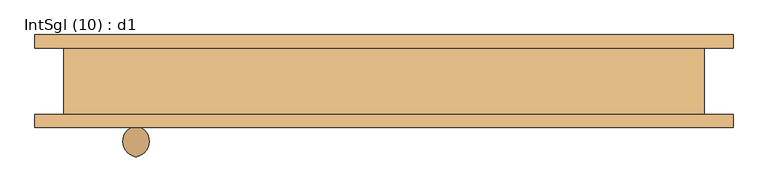
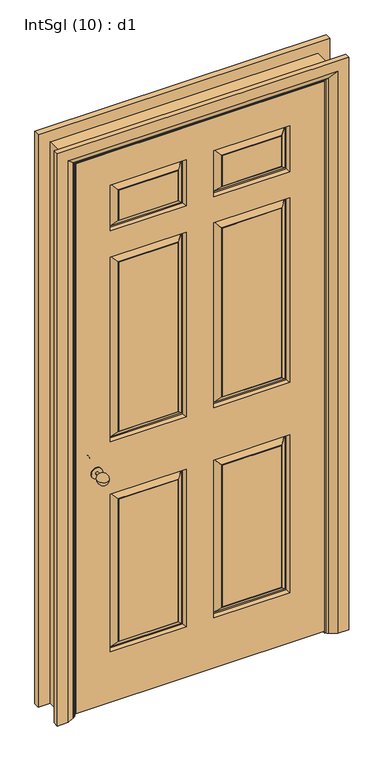
"""IFC4 building model written with IfcOpenShell, lengths in millimetres: door geometry, IntSgl (10) : d1."""

from ifc_helpers import new_model, si_unit, point, frame, origin, place, context, project, spatial, polyline, circle_curve, ellipse_curve, trimmed, outline, extrude, faceted_brep, source, transform, mapped, element, save
from ifc_brep_helpers import plane_surface, cylinder_surface, revolved_surface, advanced_brep


def intsgl_10_d1_0c106969(model_context):
    return source(origin(), model_context, "Body", "SolidModel", [
        advanced_brep(
        [(-368.0, 7.0, 900.0), (-378.0, 7.0, 900.0), (-373.0, 51.437411, 900.0), (-368.0, -8.0, 900.0), (-378.0, -8.0, 900.0), (-393.0, -12.0, 900.0), (-353.0, -12.0, 900.0), (-393.0, -8.0, 900.0), (-353.0, -8.0, 900.0)],
        [
            (0, 1, circle_curve(frame((-373.0, 7.0, 900.0), z_axis=(0.0, 1.0, 0.0), x_axis=(-1.0, 0.0, 0.0)), 5.0)),
            (1, 2, circle_curve(frame((-369.8115138, 28.5786495, 900.0), z_axis=(0.0, 0.0, -1.0), x_axis=(0.0, -1.0, 0.0)), 23.0800654)),
            (2, 0, circle_curve(frame((-376.1884862, 28.5786495, 900.0), z_axis=(0.0, 0.0, -1.0), x_axis=(0.0, -1.0, 0.0)), 23.0800654)),
            (1, 0, circle_curve(frame((-373.0, 7.0, 900.0), z_axis=(0.0, 1.0, 0.0), x_axis=(-1.0, 0.0, 0.0)), 5.0)),
            (0, 3),
            (3, 4, circle_curve(frame((-373.0, -8.0, 900.0), z_axis=(0.0, 1.0, 0.0), x_axis=(-1.0, 0.0, 0.0)), 5.0)),
            (4, 1),
            (4, 3, circle_curve(frame((-373.0, -8.0, 900.0), z_axis=(0.0, 1.0, 0.0), x_axis=(-1.0, 0.0, 0.0)), 5.0)),
            (5, 6, circle_curve(frame((-373.0, -12.0, 900.0), z_axis=(0.0, -1.0, 0.0), x_axis=(1.0, 0.0, 0.0)), 20.0)),
            (6, 5, circle_curve(frame((-373.0, -12.0, 900.0), z_axis=(0.0, -1.0, 0.0), x_axis=(1.0, 0.0, 0.0)), 20.0)),
            (7, 8, circle_curve(frame((-373.0, -8.0, 900.0), z_axis=(0.0, 1.0, 0.0), x_axis=(1.0, 0.0, 0.0)), 20.0)),
            (8, 7, circle_curve(frame((-373.0, -8.0, 900.0), z_axis=(0.0, 1.0, 0.0), x_axis=(1.0, 0.0, 0.0)), 20.0)),
            (5, 7),
            (8, 6),
        ],
        [
            revolved_surface(trimmed(ellipse_curve(frame((-369.8115138, 28.5786495, 900.0), z_axis=(0.0, 0.0, 1.0), x_axis=(0.0, -1.0, 0.0)), 23.0800654, 23.0800654), [point((-373.0, 51.437411, 900.0))], [point((-378.0, 7.0, 900.0))], True, "CARTESIAN"), (-373.0, -8.0, 900.0), (0.0, -1.0, 0.0)),
            cylinder_surface(frame((-373.0, -8.0, 900.0), z_axis=(0.0, -1.0, 0.0), x_axis=(-1.0, 0.0, 0.0)), 5.0),
            plane_surface(frame((-353.0, -12.0, 900.0), z_axis=(0.0, -1.0, 0.0), x_axis=(0.0, 0.0, 1.0))),
            plane_surface(frame((-353.0, -8.0, 900.0), z_axis=(0.0, 1.0, 0.0), x_axis=(0.0, 0.0, -1.0))),
            cylinder_surface(frame((-373.0, -8.0, 900.0), z_axis=(0.0, -1.0, 0.0), x_axis=(1.0, 0.0, 0.0)), 20.0),
        ],
        [
            (0, [[1, 2, 3]]),
            (0, [[-2, 4, -3]]),
            (1, [[-1, 5, 6, 7]]),
            (1, [[-4, -7, 8, -5]]),
            (2, [[9, 10]]),
            (3, [[11, 12], [-6, -8]]),
            (4, [[-9, 13, -12, 14]]),
            (4, [[-10, -14, -11, -13]]),
        ],
    ),
        advanced_brep(
        [(-368.0, -69.0, 900.0), (-373.0, -113.437411, 900.0), (-378.0, -69.0, 900.0), (-378.0, -54.0, 900.0), (-368.0, -54.0, 900.0), (-393.0, -50.0, 900.0), (-353.0, -50.0, 900.0), (-393.0, -54.0, 900.0), (-353.0, -54.0, 900.0)],
        [
            (0, 1, circle_curve(frame((-376.1884862, -90.5786495, 900.0), z_axis=(0.0, 0.0, -1.0), x_axis=(0.0, 1.0, 0.0)), 23.0800654)),
            (1, 2, circle_curve(frame((-369.8115138, -90.5786495, 900.0), z_axis=(0.0, 0.0, -1.0), x_axis=(0.0, 1.0, 0.0)), 23.0800654)),
            (2, 0, circle_curve(frame((-373.0, -69.0, 900.0), z_axis=(0.0, -1.0, 0.0), x_axis=(-1.0, 0.0, 0.0)), 5.0)),
            (0, 2, circle_curve(frame((-373.0, -69.0, 900.0), z_axis=(0.0, -1.0, 0.0), x_axis=(-1.0, 0.0, 0.0)), 5.0)),
            (2, 3),
            (3, 4, circle_curve(frame((-373.0, -54.0, 900.0), z_axis=(0.0, -1.0, 0.0), x_axis=(-1.0, 0.0, 0.0)), 5.0)),
            (4, 0),
            (4, 3, circle_curve(frame((-373.0, -54.0, 900.0), z_axis=(0.0, -1.0, 0.0), x_axis=(-1.0, 0.0, 0.0)), 5.0)),
            (5, 6, circle_curve(frame((-373.0, -50.0, 900.0), z_axis=(0.0, 1.0, 0.0), x_axis=(1.0, 0.0, 0.0)), 20.0)),
            (6, 5, circle_curve(frame((-373.0, -50.0, 900.0), z_axis=(0.0, 1.0, 0.0), x_axis=(1.0, 0.0, 0.0)), 20.0)),
            (7, 8, circle_curve(frame((-373.0, -54.0, 900.0), z_axis=(0.0, -1.0, 0.0), x_axis=(1.0, 0.0, 0.0)), 20.0)),
            (8, 7, circle_curve(frame((-373.0, -54.0, 900.0), z_axis=(0.0, -1.0, 0.0), x_axis=(1.0, 0.0, 0.0)), 20.0)),
            (6, 8),
            (7, 5),
        ],
        [
            revolved_surface(trimmed(ellipse_curve(frame((-369.8115138, -90.5786495, 900.0), z_axis=(0.0, 0.0, -1.0), x_axis=(0.0, 1.0, 0.0)), 23.0800654, 23.0800654), [point((-373.0, -113.437411, 900.0))], [point((-378.0, -69.0, 900.0))], True, "CARTESIAN"), (-373.0, -54.0, 900.0), (0.0, 1.0, 0.0)),
            cylinder_surface(frame((-373.0, -54.0, 900.0), z_axis=(0.0, 1.0, 0.0), x_axis=(-1.0, 0.0, 0.0)), 5.0),
            plane_surface(frame((-353.0, -50.0, 900.0), z_axis=(0.0, 1.0, 0.0), x_axis=(0.0, 0.0, 1.0))),
            plane_surface(frame((-353.0, -54.0, 900.0), z_axis=(0.0, -1.0, 0.0), x_axis=(0.0, 0.0, -1.0))),
            cylinder_surface(frame((-373.0, -54.0, 900.0), z_axis=(0.0, 1.0, 0.0), x_axis=(1.0, 0.0, 0.0)), 20.0),
        ],
        [
            (0, [[1, 2, 3]]),
            (0, [[-1, 4, -2]]),
            (1, [[5, 6, 7, -3]]),
            (1, [[-7, 8, -5, -4]]),
            (2, [[9, 10]]),
            (3, [[11, 12], [-8, -6]]),
            (4, [[13, -11, 14, -10]]),
            (4, [[-14, -12, -13, -9]]),
        ],
    ),
        faceted_brep([(-448.0, -12.0, 2103.0), (448.0, -12.0, 2103.0), (448.0, -12.0, 8.0), (-448.0, -12.0, 8.0), (-50.0, -12.0, 800.0), (-323.0, -12.0, 800.0), (-323.0, -12.0, 200.0), (-50.0, -12.0, 200.0), (323.0, -12.0, 800.0), (50.0, -12.0, 800.0), (50.0, -12.0, 200.0), (323.0, -12.0, 200.0), (-50.0, -12.0, 1703.0), (-323.0, -12.0, 1703.0), (-323.0, -12.0, 1000.0), (-50.0, -12.0, 1000.0), (323.0, -12.0, 1703.0), (50.0, -12.0, 1703.0), (50.0, -12.0, 1000.0), (323.0, -12.0, 1000.0), (-50.0, -12.0, 1978.0), (-323.0, -12.0, 1978.0), (-323.0, -12.0, 1803.0), (-50.0, -12.0, 1803.0), (323.0, -12.0, 1978.0), (50.0, -12.0, 1978.0), (50.0, -12.0, 1803.0), (323.0, -12.0, 1803.0), (-80.0, -12.0, 230.0), (-293.0, -12.0, 230.0), (-293.0, -12.0, 770.0), (-80.0, -12.0, 770.0), (293.0, -12.0, 230.0), (80.0, -12.0, 230.0), (80.0, -12.0, 770.0), (293.0, -12.0, 770.0), (-80.0, -12.0, 1030.0), (-293.0, -12.0, 1030.0), (-293.0, -12.0, 1673.0), (-80.0, -12.0, 1673.0), (293.0, -12.0, 1030.0), (80.0, -12.0, 1030.0), (80.0, -12.0, 1673.0), (293.0, -12.0, 1673.0), (-80.0, -12.0, 1833.0), (-293.0, -12.0, 1833.0), (-293.0, -12.0, 1948.0), (-80.0, -12.0, 1948.0), (293.0, -12.0, 1833.0), (80.0, -12.0, 1833.0), (80.0, -12.0, 1948.0), (293.0, -12.0, 1948.0), (-448.0, -50.0, 2103.0), (-448.0, -50.0, 8.0), (448.0, -50.0, 8.0), (448.0, -50.0, 2103.0), (50.0, -50.0, 800.0), (323.0, -50.0, 800.0), (323.0, -50.0, 200.0), (50.0, -50.0, 200.0), (-323.0, -50.0, 800.0), (-50.0, -50.0, 800.0), (-50.0, -50.0, 200.0), (-323.0, -50.0, 200.0), (50.0, -50.0, 1703.0), (323.0, -50.0, 1703.0), (323.0, -50.0, 1000.0), (50.0, -50.0, 1000.0), (-323.0, -50.0, 1703.0), (-50.0, -50.0, 1703.0), (-50.0, -50.0, 1000.0), (-323.0, -50.0, 1000.0), (50.0, -50.0, 1978.0), (323.0, -50.0, 1978.0), (323.0, -50.0, 1803.0), (50.0, -50.0, 1803.0), (-323.0, -50.0, 1978.0), (-50.0, -50.0, 1978.0), (-50.0, -50.0, 1803.0), (-323.0, -50.0, 1803.0), (80.0, -50.0, 230.0), (293.0, -50.0, 230.0), (293.0, -50.0, 770.0), (80.0, -50.0, 770.0), (-293.0, -50.0, 230.0), (-80.0, -50.0, 230.0), (-80.0, -50.0, 770.0), (-293.0, -50.0, 770.0), (80.0, -50.0, 1030.0), (293.0, -50.0, 1030.0), (293.0, -50.0, 1673.0), (80.0, -50.0, 1673.0), (-293.0, -50.0, 1030.0), (-80.0, -50.0, 1030.0), (-80.0, -50.0, 1673.0), (-293.0, -50.0, 1673.0), (80.0, -50.0, 1833.0), (293.0, -50.0, 1833.0), (293.0, -50.0, 1948.0), (80.0, -50.0, 1948.0), (-293.0, -50.0, 1833.0), (-80.0, -50.0, 1833.0), (-80.0, -50.0, 1948.0), (-293.0, -50.0, 1948.0), (80.0, -49.0, 230.0), (80.0, -49.0, 770.0), (58.0, -35.0, 208.0), (78.0, -49.0, 228.0), (78.0, -49.0, 772.0), (58.0, -35.0, 792.0), (53.0, -35.0, 203.0), (53.0, -35.0, 797.0), (293.0, -49.0, 770.0), (295.0, -49.0, 772.0), (315.0, -35.0, 792.0), (320.0, -35.0, 797.0), (293.0, -49.0, 230.0), (295.0, -49.0, 228.0), (315.0, -35.0, 208.0), (320.0, -35.0, 203.0), (-293.0, -49.0, 230.0), (-293.0, -49.0, 770.0), (-315.0, -35.0, 208.0), (-295.0, -49.0, 228.0), (-295.0, -49.0, 772.0), (-315.0, -35.0, 792.0), (-320.0, -35.0, 203.0), (-320.0, -35.0, 797.0), (-80.0, -49.0, 770.0), (-78.0, -49.0, 772.0), (-58.0, -35.0, 792.0), (-53.0, -35.0, 797.0), (-80.0, -49.0, 230.0), (-78.0, -49.0, 228.0), (-58.0, -35.0, 208.0), (-53.0, -35.0, 203.0), (80.0, -49.0, 1030.0), (80.0, -49.0, 1673.0), (58.0, -35.0, 1008.0), (78.0, -49.0, 1028.0), (78.0, -49.0, 1675.0), (58.0, -35.0, 1695.0), (53.0, -35.0, 1003.0), (53.0, -35.0, 1700.0), (293.0, -49.0, 1673.0), (295.0, -49.0, 1675.0), (315.0, -35.0, 1695.0), (320.0, -35.0, 1700.0), (293.0, -49.0, 1030.0), (295.0, -49.0, 1028.0), (315.0, -35.0, 1008.0), (320.0, -35.0, 1003.0), (-293.0, -49.0, 1030.0), (-293.0, -49.0, 1673.0), (-315.0, -35.0, 1008.0), (-295.0, -49.0, 1028.0), (-295.0, -49.0, 1675.0), (-315.0, -35.0, 1695.0), (-320.0, -35.0, 1003.0), (-320.0, -35.0, 1700.0), (-80.0, -49.0, 1673.0), (-78.0, -49.0, 1675.0), (-58.0, -35.0, 1695.0), (-53.0, -35.0, 1700.0), (-80.0, -49.0, 1030.0), (-78.0, -49.0, 1028.0), (-58.0, -35.0, 1008.0), (-53.0, -35.0, 1003.0), (80.0, -49.0, 1833.0), (80.0, -49.0, 1948.0), (58.0, -35.0, 1811.0), (78.0, -49.0, 1831.0), (78.0, -49.0, 1950.0), (58.0, -35.0, 1970.0), (53.0, -35.0, 1806.0), (53.0, -35.0, 1975.0), (293.0, -49.0, 1948.0), (295.0, -49.0, 1950.0), (315.0, -35.0, 1970.0), (320.0, -35.0, 1975.0), (293.0, -49.0, 1833.0), (295.0, -49.0, 1831.0), (315.0, -35.0, 1811.0), (320.0, -35.0, 1806.0), (-293.0, -49.0, 1833.0), (-293.0, -49.0, 1948.0), (-315.0, -35.0, 1811.0), (-295.0, -49.0, 1831.0), (-295.0, -49.0, 1950.0), (-315.0, -35.0, 1970.0), (-320.0, -35.0, 1806.0), (-320.0, -35.0, 1975.0), (-80.0, -49.0, 1948.0), (-78.0, -49.0, 1950.0), (-58.0, -35.0, 1970.0), (-53.0, -35.0, 1975.0), (-80.0, -49.0, 1833.0), (-78.0, -49.0, 1831.0), (-58.0, -35.0, 1811.0), (-53.0, -35.0, 1806.0), (-80.0, -13.0, 230.0), (-80.0, -13.0, 770.0), (-58.0, -27.0, 208.0), (-78.0, -13.0, 228.0), (-78.0, -13.0, 772.0), (-58.0, -27.0, 792.0), (-53.0, -27.0, 203.0), (-53.0, -27.0, 797.0), (-293.0, -13.0, 770.0), (-295.0, -13.0, 772.0), (-315.0, -27.0, 792.0), (-320.0, -27.0, 797.0), (-293.0, -13.0, 230.0), (-295.0, -13.0, 228.0), (-315.0, -27.0, 208.0), (-320.0, -27.0, 203.0), (293.0, -13.0, 230.0), (293.0, -13.0, 770.0), (315.0, -27.0, 208.0), (295.0, -13.0, 228.0), (295.0, -13.0, 772.0), (315.0, -27.0, 792.0), (320.0, -27.0, 203.0), (320.0, -27.0, 797.0), (80.0, -13.0, 770.0), (78.0, -13.0, 772.0), (58.0, -27.0, 792.0), (53.0, -27.0, 797.0), (80.0, -13.0, 230.0), (78.0, -13.0, 228.0), (58.0, -27.0, 208.0), (53.0, -27.0, 203.0), (-80.0, -13.0, 1030.0), (-80.0, -13.0, 1673.0), (-58.0, -27.0, 1008.0), (-78.0, -13.0, 1028.0), (-78.0, -13.0, 1675.0), (-58.0, -27.0, 1695.0), (-53.0, -27.0, 1003.0), (-53.0, -27.0, 1700.0), (-293.0, -13.0, 1673.0), (-295.0, -13.0, 1675.0), (-315.0, -27.0, 1695.0), (-320.0, -27.0, 1700.0), (-293.0, -13.0, 1030.0), (-295.0, -13.0, 1028.0), (-315.0, -27.0, 1008.0), (-320.0, -27.0, 1003.0), (293.0, -13.0, 1030.0), (293.0, -13.0, 1673.0), (315.0, -27.0, 1008.0), (295.0, -13.0, 1028.0), (295.0, -13.0, 1675.0), (315.0, -27.0, 1695.0), (320.0, -27.0, 1003.0), (320.0, -27.0, 1700.0), (80.0, -13.0, 1673.0), (78.0, -13.0, 1675.0), (58.0, -27.0, 1695.0), (53.0, -27.0, 1700.0), (80.0, -13.0, 1030.0), (78.0, -13.0, 1028.0), (58.0, -27.0, 1008.0), (53.0, -27.0, 1003.0), (-80.0, -13.0, 1833.0), (-80.0, -13.0, 1948.0), (-58.0, -27.0, 1811.0), (-78.0, -13.0, 1831.0), (-78.0, -13.0, 1950.0), (-58.0, -27.0, 1970.0), (-53.0, -27.0, 1806.0), (-53.0, -27.0, 1975.0), (-293.0, -13.0, 1948.0), (-295.0, -13.0, 1950.0), (-315.0, -27.0, 1970.0), (-320.0, -27.0, 1975.0), (-293.0, -13.0, 1833.0), (-295.0, -13.0, 1831.0), (-315.0, -27.0, 1811.0), (-320.0, -27.0, 1806.0), (293.0, -13.0, 1833.0), (293.0, -13.0, 1948.0), (315.0, -27.0, 1811.0), (295.0, -13.0, 1831.0), (295.0, -13.0, 1950.0), (315.0, -27.0, 1970.0), (320.0, -27.0, 1806.0), (320.0, -27.0, 1975.0), (80.0, -13.0, 1948.0), (78.0, -13.0, 1950.0), (58.0, -27.0, 1970.0), (53.0, -27.0, 1975.0), (80.0, -13.0, 1833.0), (78.0, -13.0, 1831.0), (58.0, -27.0, 1811.0), (53.0, -27.0, 1806.0)], [[[0, 1, 2, 3], [4, 5, 6, 7], [8, 9, 10, 11], [12, 13, 14, 15], [16, 17, 18, 19], [20, 21, 22, 23], [24, 25, 26, 27]], [[28, 29, 30, 31]], [[32, 33, 34, 35]], [[36, 37, 38, 39]], [[40, 41, 42, 43]], [[44, 45, 46, 47]], [[48, 49, 50, 51]], [[52, 53, 54, 55], [56, 57, 58, 59], [60, 61, 62, 63], [64, 65, 66, 67], [68, 69, 70, 71], [72, 73, 74, 75], [76, 77, 78, 79]], [[80, 81, 82, 83]], [[84, 85, 86, 87]], [[88, 89, 90, 91]], [[92, 93, 94, 95]], [[96, 97, 98, 99]], [[100, 101, 102, 103]], [[3, 53, 52, 0]], [[2, 54, 53, 3]], [[1, 55, 54, 2]], [[0, 52, 55, 1]], [[104, 80, 83, 105]], [[106, 107, 108, 109]], [[56, 59, 110, 111]], [[83, 82, 112, 105]], [[108, 113, 114, 109]], [[111, 115, 57, 56]], [[82, 81, 116, 112]], [[113, 117, 118, 114]], [[115, 119, 58, 57]], [[104, 116, 81, 80]], [[107, 117, 113, 108], [105, 112, 116, 104]], [[106, 118, 117, 107]], [[110, 119, 115, 111], [109, 114, 118, 106]], [[59, 58, 119, 110]], [[120, 84, 87, 121]], [[122, 123, 124, 125]], [[60, 63, 126, 127]], [[87, 86, 128, 121]], [[124, 129, 130, 125]], [[127, 131, 61, 60]], [[86, 85, 132, 128]], [[129, 133, 134, 130]], [[131, 135, 62, 61]], [[120, 132, 85, 84]], [[123, 133, 129, 124], [121, 128, 132, 120]], [[122, 134, 133, 123]], [[126, 135, 131, 127], [125, 130, 134, 122]], [[63, 62, 135, 126]], [[136, 88, 91, 137]], [[138, 139, 140, 141]], [[64, 67, 142, 143]], [[91, 90, 144, 137]], [[140, 145, 146, 141]], [[143, 147, 65, 64]], [[90, 89, 148, 144]], [[145, 149, 150, 146]], [[147, 151, 66, 65]], [[136, 148, 89, 88]], [[139, 149, 145, 140], [137, 144, 148, 136]], [[138, 150, 149, 139]], [[142, 151, 147, 143], [141, 146, 150, 138]], [[67, 66, 151, 142]], [[152, 92, 95, 153]], [[154, 155, 156, 157]], [[68, 71, 158, 159]], [[95, 94, 160, 153]], [[156, 161, 162, 157]], [[159, 163, 69, 68]], [[94, 93, 164, 160]], [[161, 165, 166, 162]], [[163, 167, 70, 69]], [[152, 164, 93, 92]], [[155, 165, 161, 156], [153, 160, 164, 152]], [[154, 166, 165, 155]], [[158, 167, 163, 159], [157, 162, 166, 154]], [[71, 70, 167, 158]], [[168, 96, 99, 169]], [[170, 171, 172, 173]], [[72, 75, 174, 175]], [[99, 98, 176, 169]], [[172, 177, 178, 173]], [[175, 179, 73, 72]], [[98, 97, 180, 176]], [[177, 181, 182, 178]], [[179, 183, 74, 73]], [[168, 180, 97, 96]], [[171, 181, 177, 172], [169, 176, 180, 168]], [[170, 182, 181, 171]], [[174, 183, 179, 175], [173, 178, 182, 170]], [[75, 74, 183, 174]], [[184, 100, 103, 185]], [[186, 187, 188, 189]], [[76, 79, 190, 191]], [[103, 102, 192, 185]], [[188, 193, 194, 189]], [[191, 195, 77, 76]], [[102, 101, 196, 192]], [[193, 197, 198, 194]], [[195, 199, 78, 77]], [[184, 196, 101, 100]], [[187, 197, 193, 188], [185, 192, 196, 184]], [[186, 198, 197, 187]], [[190, 199, 195, 191], [189, 194, 198, 186]], [[79, 78, 199, 190]], [[200, 28, 31, 201]], [[202, 203, 204, 205]], [[4, 7, 206, 207]], [[31, 30, 208, 201]], [[204, 209, 210, 205]], [[207, 211, 5, 4]], [[30, 29, 212, 208]], [[209, 213, 214, 210]], [[211, 215, 6, 5]], [[200, 212, 29, 28]], [[203, 213, 209, 204], [201, 208, 212, 200]], [[202, 214, 213, 203]], [[206, 215, 211, 207], [205, 210, 214, 202]], [[7, 6, 215, 206]], [[216, 32, 35, 217]], [[218, 219, 220, 221]], [[8, 11, 222, 223]], [[35, 34, 224, 217]], [[220, 225, 226, 221]], [[223, 227, 9, 8]], [[34, 33, 228, 224]], [[225, 229, 230, 226]], [[227, 231, 10, 9]], [[216, 228, 33, 32]], [[219, 229, 225, 220], [217, 224, 228, 216]], [[218, 230, 229, 219]], [[222, 231, 227, 223], [221, 226, 230, 218]], [[11, 10, 231, 222]], [[232, 36, 39, 233]], [[234, 235, 236, 237]], [[12, 15, 238, 239]], [[39, 38, 240, 233]], [[236, 241, 242, 237]], [[239, 243, 13, 12]], [[38, 37, 244, 240]], [[241, 245, 246, 242]], [[243, 247, 14, 13]], [[232, 244, 37, 36]], [[235, 245, 241, 236], [233, 240, 244, 232]], [[234, 246, 245, 235]], [[238, 247, 243, 239], [237, 242, 246, 234]], [[15, 14, 247, 238]], [[248, 40, 43, 249]], [[250, 251, 252, 253]], [[16, 19, 254, 255]], [[43, 42, 256, 249]], [[252, 257, 258, 253]], [[255, 259, 17, 16]], [[42, 41, 260, 256]], [[257, 261, 262, 258]], [[259, 263, 18, 17]], [[248, 260, 41, 40]], [[251, 261, 257, 252], [249, 256, 260, 248]], [[250, 262, 261, 251]], [[254, 263, 259, 255], [253, 258, 262, 250]], [[19, 18, 263, 254]], [[264, 44, 47, 265]], [[266, 267, 268, 269]], [[20, 23, 270, 271]], [[47, 46, 272, 265]], [[268, 273, 274, 269]], [[271, 275, 21, 20]], [[46, 45, 276, 272]], [[273, 277, 278, 274]], [[275, 279, 22, 21]], [[264, 276, 45, 44]], [[267, 277, 273, 268], [265, 272, 276, 264]], [[266, 278, 277, 267]], [[270, 279, 275, 271], [269, 274, 278, 266]], [[23, 22, 279, 270]], [[280, 48, 51, 281]], [[282, 283, 284, 285]], [[24, 27, 286, 287]], [[51, 50, 288, 281]], [[284, 289, 290, 285]], [[287, 291, 25, 24]], [[50, 49, 292, 288]], [[289, 293, 294, 290]], [[291, 295, 26, 25]], [[280, 292, 49, 48]], [[283, 293, 289, 284], [281, 288, 292, 280]], [[282, 294, 293, 283]], [[286, 295, 291, 287], [285, 290, 294, 282]], [[27, 26, 295, 286]]]),
        advanced_brep(
        [(525.0, -70.0, 0.0), (485.0, -70.0, 0.0), (459.0, -56.0, 0.0), (455.0, -50.0, 0.0), (525.0, -50.0, 0.0), (525.0, -50.0, 2180.0), (525.0, -70.0, 2180.0), (455.0, -50.0, 2110.0), (-455.0, -50.0, 2110.0), (-455.0, -50.0, 0.0), (-525.0, -50.0, 0.0), (-525.0, -50.0, 2180.0), (459.0, -56.0, 2114.0), (485.0, -70.0, 2140.0), (-525.0, -70.0, 2180.0), (-525.0, -70.0, 0.0), (-485.0, -70.0, 0.0), (-485.0, -70.0, 2140.0), (-459.0, -56.0, 0.0), (-459.0, -56.0, 2114.0)],
        [
            (0, 1),
            (1, 2),
            (2, 3, circle_curve(frame((463.0, -49.0, 0.0), z_axis=(0.0, 0.0, -1.0), x_axis=(1.0, 0.0, 0.0)), 8.0622577)),
            (3, 4),
            (4, 0),
            (4, 5),
            (5, 6),
            (6, 0),
            (3, 7),
            (7, 8),
            (8, 9),
            (9, 10),
            (10, 11),
            (11, 5),
            (2, 12),
            (12, 7, ellipse_curve(frame((463.0, -49.0, 2118.0), z_axis=(0.7071067811865475, 0.0, -0.7071067811865475), x_axis=(-0.7071067811865474, 0.0, -0.7071067811865476)), 11.4017543, 8.0622577)),
            (1, 13),
            (13, 12),
            (6, 14),
            (14, 15),
            (15, 16),
            (16, 17),
            (17, 13),
            (10, 15),
            (14, 11),
            (9, 18, circle_curve(frame((-463.0, -49.0, 0.0), z_axis=(0.0, 0.0, -1.0), x_axis=(-1.0, 0.0, 0.0)), 8.0622577)),
            (18, 16),
            (19, 18),
            (8, 19, ellipse_curve(frame((-463.0, -49.0, 2118.0), z_axis=(-0.7071067811865475, 0.0, -0.7071067811865475), x_axis=(-0.7071067811865474, 0.0, 0.7071067811865476)), 11.4017543, 8.0622577)),
            (19, 17),
            (12, 19),
        ],
        [
            plane_surface(frame((455.0, -50.0, 0.0), z_axis=(0.0, 0.0, -1.0), x_axis=(0.0, -1.0, 0.0))),
            plane_surface(frame((525.0, -70.0, 0.0), z_axis=(1.0, 0.0, 0.0), x_axis=(0.0, 0.0, 1.0))),
            plane_surface(frame((525.0, -50.0, 0.0), z_axis=(0.0, 1.0, 0.0), x_axis=(0.0, 0.0, 1.0))),
            cylinder_surface(frame((463.0, -49.0, 0.0), z_axis=(0.0, 0.0, -1.0), x_axis=(1.0, 0.0, 0.0)), 8.0622577),
            plane_surface(frame((459.0, -56.0, 0.0), z_axis=(-0.4740998230350183, -0.8804710999221749, 0.0), x_axis=(0.0, 0.0, 1.0))),
            plane_surface(frame((485.0, -70.0, 0.0), z_axis=(0.0, -1.0, 0.0), x_axis=(0.0, 0.0, 1.0))),
            plane_surface(frame((-525.0, -70.0, 2180.0), z_axis=(-1.0, 0.0, 0.0), x_axis=(0.0, 0.0, -1.0))),
            plane_surface(frame((-455.0, -50.0, 0.0), z_axis=(0.0, 0.0, -1.0), x_axis=(0.0, -1.0, 0.0))),
            cylinder_surface(frame((-463.0, -49.0, 2110.0), z_axis=(0.0, 0.0, 1.0), x_axis=(-1.0, 0.0, 0.0)), 8.0622577),
            plane_surface(frame((-459.0, -56.0, 2114.0), z_axis=(0.4740998230350183, -0.8804710999221749, 0.0), x_axis=(0.0, 0.0, -1.0))),
            plane_surface(frame((525.0, -70.0, 2180.0), z_axis=(0.0, 0.0, 1.0), x_axis=(-1.0, 0.0, 0.0))),
            cylinder_surface(frame((455.0, -49.0, 2118.0), z_axis=(1.0, 0.0, 0.0), x_axis=(0.0, 0.0, 1.0)), 8.0622577),
            plane_surface(frame((459.0, -56.0, 2114.0), z_axis=(0.0, -0.8804710999221749, -0.4740998230350183), x_axis=(-1.0, 0.0, 0.0))),
        ],
        [
            (0, [[1, 2, 3, 4, 5]]),
            (1, [[6, 7, 8, -5]]),
            (2, [[9, 10, 11, 12, 13, 14, -6, -4]]),
            (3, [[15, 16, -9, -3]]),
            (4, [[17, 18, -15, -2]]),
            (5, [[-8, 19, 20, 21, 22, 23, -17, -1]]),
            (6, [[-13, 24, -20, 25]]),
            (7, [[-24, -12, 26, 27, -21]]),
            (8, [[28, -26, -11, 29]]),
            (9, [[-22, -27, -28, 30]]),
            (10, [[-14, -25, -19, -7]]),
            (11, [[31, -29, -10, -16]]),
            (12, [[-23, -30, -31, -18]]),
        ],
    ),
        advanced_brep(
        [(-525.0, 70.0, 0.0), (-485.0, 70.0, 0.0), (-459.0, 56.0, 0.0), (-455.0, 50.0, 0.0), (-525.0, 50.0, 0.0), (-525.0, 50.0, 2180.0), (-525.0, 70.0, 2180.0), (-455.0, 50.0, 2110.0), (455.0, 50.0, 2110.0), (455.0, 50.0, 0.0), (525.0, 50.0, 0.0), (525.0, 50.0, 2180.0), (-459.0, 56.0, 2114.0), (-485.0, 70.0, 2140.0), (525.0, 70.0, 2180.0), (525.0, 70.0, 0.0), (485.0, 70.0, 0.0), (485.0, 70.0, 2140.0), (459.0, 56.0, 0.0), (459.0, 56.0, 2114.0)],
        [
            (0, 1),
            (1, 2),
            (2, 3, circle_curve(frame((-463.0, 49.0, 0.0), z_axis=(0.0, 0.0, -1.0), x_axis=(-1.0, 0.0, 0.0)), 8.0622577)),
            (3, 4),
            (4, 0),
            (4, 5),
            (5, 6),
            (6, 0),
            (3, 7),
            (7, 8),
            (8, 9),
            (9, 10),
            (10, 11),
            (11, 5),
            (2, 12),
            (12, 7, ellipse_curve(frame((-463.0, 49.0, 2118.0), z_axis=(-0.7071067811865475, 0.0, -0.7071067811865475), x_axis=(0.7071067811865474, 0.0, -0.7071067811865476)), 11.4017543, 8.0622577)),
            (1, 13),
            (13, 12),
            (6, 14),
            (14, 15),
            (15, 16),
            (16, 17),
            (17, 13),
            (10, 15),
            (14, 11),
            (9, 18, circle_curve(frame((463.0, 49.0, 0.0), z_axis=(0.0, 0.0, -1.0), x_axis=(1.0, 0.0, 0.0)), 8.0622577)),
            (18, 16),
            (19, 18),
            (8, 19, ellipse_curve(frame((463.0, 49.0, 2118.0), z_axis=(0.7071067811865475, 0.0, -0.7071067811865475), x_axis=(0.7071067811865474, 0.0, 0.7071067811865476)), 11.4017543, 8.0622577)),
            (19, 17),
            (12, 19),
        ],
        [
            plane_surface(frame((-455.0, 50.0, 0.0), z_axis=(0.0, 0.0, -1.0), x_axis=(0.0, 1.0, 0.0))),
            plane_surface(frame((-525.0, 70.0, 0.0), z_axis=(-1.0, 0.0, 0.0), x_axis=(0.0, 0.0, 1.0))),
            plane_surface(frame((-525.0, 50.0, 0.0), z_axis=(0.0, -1.0, 0.0), x_axis=(0.0, 0.0, 1.0))),
            cylinder_surface(frame((-463.0, 49.0, 0.0), z_axis=(0.0, 0.0, -1.0), x_axis=(-1.0, 0.0, 0.0)), 8.0622577),
            plane_surface(frame((-459.0, 56.0, 0.0), z_axis=(0.4740998230350183, 0.8804710999221749, 0.0), x_axis=(0.0, 0.0, 1.0))),
            plane_surface(frame((-485.0, 70.0, 0.0), z_axis=(0.0, 1.0, 0.0), x_axis=(0.0, 0.0, 1.0))),
            plane_surface(frame((525.0, 70.0, 2180.0), z_axis=(1.0, 0.0, 0.0), x_axis=(0.0, 0.0, -1.0))),
            plane_surface(frame((455.0, 50.0, 0.0), z_axis=(0.0, 0.0, -1.0), x_axis=(0.0, 1.0, 0.0))),
            cylinder_surface(frame((463.0, 49.0, 2110.0), z_axis=(0.0, 0.0, 1.0), x_axis=(1.0, 0.0, 0.0)), 8.0622577),
            plane_surface(frame((459.0, 56.0, 2114.0), z_axis=(-0.4740998230350183, 0.8804710999221749, 0.0), x_axis=(0.0, 0.0, -1.0))),
            plane_surface(frame((-525.0, 70.0, 2180.0), z_axis=(0.0, 0.0, 1.0), x_axis=(1.0, 0.0, 0.0))),
            cylinder_surface(frame((-455.0, 49.0, 2118.0), z_axis=(-1.0, 0.0, 0.0), x_axis=(0.0, 0.0, 1.0)), 8.0622577),
            plane_surface(frame((-459.0, 56.0, 2114.0), z_axis=(0.0, 0.8804710999221749, -0.4740998230350183), x_axis=(1.0, 0.0, 0.0))),
        ],
        [
            (0, [[1, 2, 3, 4, 5]]),
            (1, [[6, 7, 8, -5]]),
            (2, [[9, 10, 11, 12, 13, 14, -6, -4]]),
            (3, [[15, 16, -9, -3]]),
            (4, [[17, 18, -15, -2]]),
            (5, [[-8, 19, 20, 21, 22, 23, -17, -1]]),
            (6, [[-13, 24, -20, 25]]),
            (7, [[-24, -12, 26, 27, -21]]),
            (8, [[28, -26, -11, 29]]),
            (9, [[-22, -27, -28, 30]]),
            (10, [[-14, -25, -19, -7]]),
            (11, [[31, -29, -10, -16]]),
            (12, [[-23, -30, -31, -18]]),
        ],
    ),
        extrude(outline(polyline([(0.0, -431.0), (2086.0, -431.0), (2086.0, 431.0), (0.0, 431.0), (0.0, 450.0), (2105.0, 450.0), (2105.0, -450.0), (0.0, -450.0), (0.0, -431.0)])), frame((0.0, -10.0, 0.0), z_axis=(0.0, 1.0, 0.0), x_axis=(0.0, 0.0, 1.0)), (0.0, 0.0, 1.0), 32.0),
        faceted_brep([(-450.0, -50.0, 0.0), (-482.0, -50.0, 0.0), (-482.0, 50.0, 0.0), (-450.0, 50.0, 0.0), (-450.0, 50.0, 2105.0), (-450.0, -50.0, 2105.0), (-482.0, 50.0, 2137.0), (-482.0, -50.0, 2137.0), (450.0, -50.0, 0.0), (450.0, 50.0, 0.0), (482.0, 50.0, 0.0), (482.0, -50.0, 0.0), (450.0, -50.0, 2105.0), (482.0, -50.0, 2137.0), (482.0, 50.0, 2137.0), (450.0, 50.0, 2105.0)], [[[0, 1, 2, 3]], [[3, 4, 5, 0]], [[2, 6, 4, 3]], [[1, 7, 6, 2]], [[0, 5, 7, 1]], [[8, 9, 10, 11]], [[12, 8, 11, 13]], [[13, 11, 10, 14]], [[14, 10, 9, 15]], [[15, 9, 8, 12]], [[4, 15, 12, 5]], [[6, 14, 15, 4]], [[7, 13, 14, 6]], [[5, 12, 13, 7]]]),
    ])


if __name__ == "__main__":
    model = new_model("IFC4")
    model_context = context("Model", 3, world=origin())
    ifc_project = project(units=[si_unit("LENGTHUNIT", "METRE", prefix="MILLI")], contexts=[model_context])
    site = spatial("IfcSite", under=ifc_project)
    building = spatial("IfcBuilding", under=site)
    placement = place(None, origin())
    intsgl_10_d1_shape = intsgl_10_d1_0c106969(model_context)
    element("IfcDoor", 1, ObjectType="IntSgl (10) : d1", at=placement, inside=building, context=model_context, shape_type="MappedRepresentation", body=[
        mapped(intsgl_10_d1_shape, transform((0.0, 0.0, 0.0), x_axis=(1.0, 0.0, 0.0), y_axis=(0.0, 1.0, 0.0), z_axis=(0.0, 0.0, 1.0))),
    ])
    save(model, "model.ifc")

# Revit data of these elements
# Type "IntSgl (10) : d1"
#   Type Mark = "11"
#   Type Comments = "Internal Single"
#   Operation = "SingleSwingRight"
#   Manufacturer = "Revit"
#   Keynote = "L20"
#   Description = "Internal Single Door"
#   UnderCut = 8 mm
#   Tolerance = 2 mm
#   Thickness = 38 mm
#   Structural Tolerance = 8 mm
#   StopDepth = 32 mm
#   Stop Thickness = 19 mm
#   Stile Top Rail = 125 mm
#   Stile Shutting = 125 mm
#   Stile Muntin Rail = 100 mm
#   Stile Lock Rail = 200 mm
#   Stile Intermediate/Frieze = 100 mm
#   Stile Hanging = 125 mm
#   Stile Bottom Rail = 200 mm
#   Rough Width = 980 mm
#   Rough Height = 2145 mm
#   Height to Top Lock Rail = 1000 mm
#   Handle Z Distance = 900 mm
#   Handle X Distance = 75 mm
#   Frame Thickness = 32 mm
#   Door Panel Width = 896 mm
#   Height = 2145 mm
#   Width = 980 mm
#   Door Panel Thickness = 38 mm
#   Door Panel Offset = 0 mm
#   Door Panel Height = 2095 mm
#   Architrave Setback = 5 mm
#   Vis - Ironmongery = yes
#   Material Ironmongery = Door - Handle
#   Material Frame = Door - Frame/Mullion
#   Material Door = Door - Panel
#   Material Architrave = Door - Architrave
#   Function = (empty or 0)
#   Wall Closure = (empty or 0)
# Element 1 (IfcDoor, "IntSgl (10) : d1")
#   Materials on its faces: "Door - Panel", "Door - Architrave", "Door - Frame/Mullion", "Door - Handle"
# Materials
#   "Door - Handle": class "Miscellaneous", colour RGB 247 247 247, transparency 0
#   "Door - Frame/Mullion": class "Wood", colour RGB 212 179 113, transparency 0
#   "Door - Panel": class "Wood", colour RGB 210 159 95, transparency 0
#   "Door - Architrave": class "Wood", colour RGB 154 90 5, transparency 0
